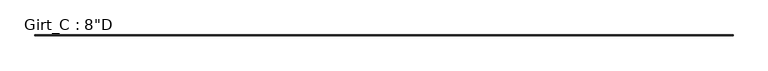
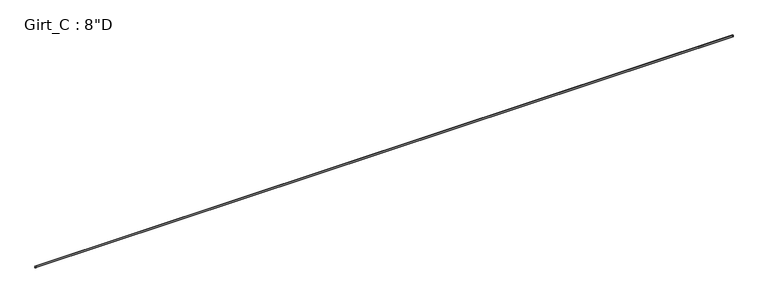
"""IFC4 building model written with IfcOpenShell, lengths in millimetres: beam geometry."""

from ifc_helpers import new_model, si_unit, point, frame, frame_2d, origin, place, context, project, spatial, polyline, circle_curve, trimmed, segment, composite_curve, outline, extrude, source, transform, mapped, element, save


def beam_83977cdd(model_context):
    return source(origin(), model_context, "Body", "SweptSolid", [
        extrude(outline(composite_curve([segment(polyline([(87.5109375, 101.6), (99.7560415, 87.0068534), (97.6278742, 85.221109), (86.2154765, 98.821875), (3.3005807, 98.821875)]), True, "CONTINUOUS"), segment(trimmed(circle_curve(frame_2d((3.3741066, 96.8381931)), 1.9850441), [point((3.3005807, 98.821875))], [point((1.3890625, 96.8381931))], True, "CARTESIAN"), True, "CONTINUOUS"), segment(polyline([(1.3890625, 96.8381931), (1.3890625, -96.8389339)]), True, "CONTINUOUS"), segment(trimmed(circle_curve(frame_2d((3.3748024, -96.8389339)), 1.9857399), [point((1.3890625, -96.8389339))], [point((3.2694106, -98.821875))], True, "CARTESIAN"), True, "CONTINUOUS"), segment(polyline([(3.2694106, -98.821875), (86.2154765, -98.821875), (97.6510975, -85.1934327), (99.7792647, -86.979177), (87.5109375, -101.6), (3.3734375, -101.6)]), True, "CONTINUOUS"), segment(trimmed(circle_curve(frame_2d((3.3734375, -96.8375)), 4.7625), [point((3.3734375, -101.6))], [point((-1.3890625, -96.8375))], False, "CARTESIAN"), True, "CONTINUOUS"), segment(polyline([(-1.3890625, -96.8375), (-1.3890625, 96.8375)]), True, "CONTINUOUS"), segment(trimmed(circle_curve(frame_2d((3.3734375, 96.8375)), 4.7625), [point((-1.3890625, 96.8375))], [point((3.3734375, 101.6))], False, "CARTESIAN"), True, "CONTINUOUS"), segment(polyline([(3.3734375, 101.6), (87.5109375, 101.6)]), True, "CONTINUOUS")], self_intersect=False)), frame((-44129.1086819, 0.0, 0.0), z_axis=(1.0, 0.0, 0.0), x_axis=(0.0, 1.0, 0.0)), (0.0, 0.0, 1.0), 88258.2173639),
    ])


if __name__ == "__main__":
    model = new_model("IFC4")
    model_context = context("Model", 3, world=origin())
    ifc_project = project(units=[si_unit("LENGTHUNIT", "METRE", prefix="MILLI")], contexts=[model_context])
    site = spatial("IfcSite", under=ifc_project)
    building = spatial("IfcBuilding", under=site)
    placement = place(None, origin())
    beam_shape = beam_83977cdd(model_context)
    element("IfcBeam", 1, ObjectType="Girt_C : 8\"D", at=placement, inside=building, context=model_context, shape_type="MappedRepresentation", body=[
        mapped(beam_shape, transform((0.0, 0.0, 0.0), x_axis=(1.0, 0.0, 0.0), y_axis=(0.0, 1.0, 0.0), z_axis=(0.0, 0.0, 1.0))),
    ])
    save(model, "model.ifc")

# Revit data of these elements
# Type "Girt_C : 8\"D"
#   half leg = 0' - 1 3/4"
#   Web_Thickness = 0' - 0 7/64"
#   Length [instance default] = 10' - 0"
#   Leg_1 = 0' - 3 1/2"
#   Height = 0' - 8"
#   Structural Material [instance default] = none
# Element 1 (IfcBeam, "Girt_C : 8\"D")
#   Structural Material = CEE' SECTION (8.0x3.5C - SEE STRUCT. DWGS)
#   Materials on its faces: "CEE' SECTION (8.0x3.5C - SEE STRUCT. DWGS)"
# Materials
#   "CEE' SECTION (8.0x3.5C - SEE STRUCT. DWGS)": class "Metal", colour RGB 137 146 153, transparency 0, Description = "Steel, mill finish", Cost = 0
